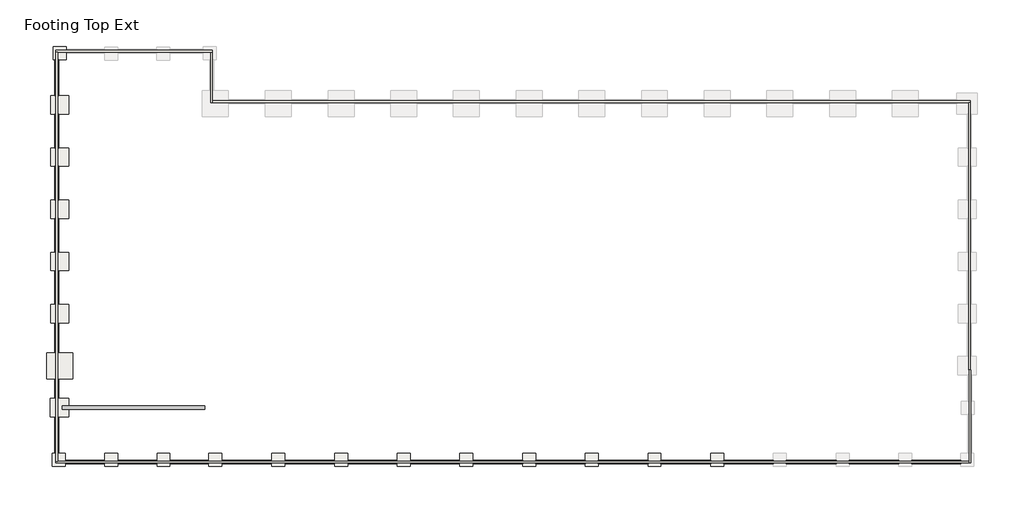
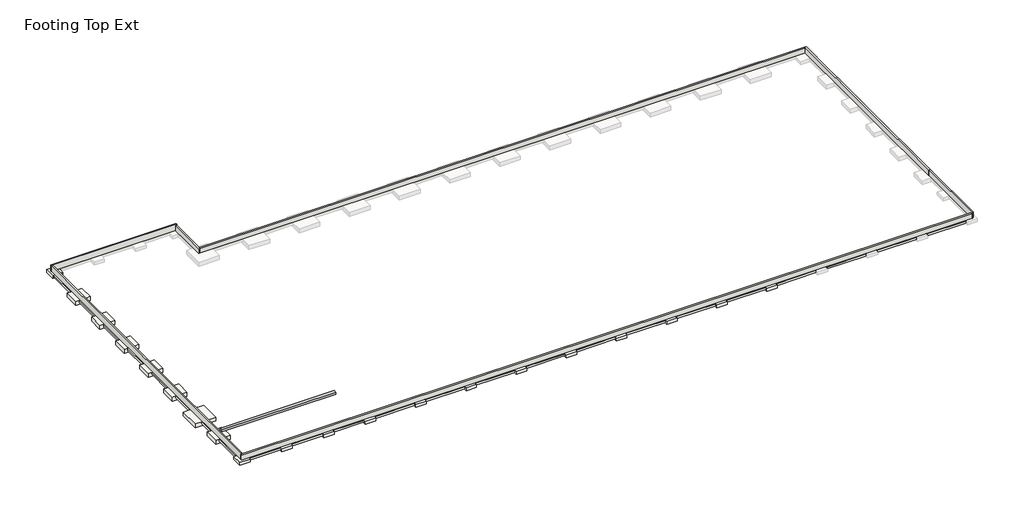
# One storey, part 1 of 2: 20 slabs, 7 walls, 2 footings, 1 beam.
"""IFC4 building model written with IfcOpenShell, lengths in millimetres."""

from ifc_helpers import new_model, si_unit, frame, origin, place, context, project, spatial, polyline, outline, extrude, faceted_brep, element, save

model = new_model("IFC4")

# Units and contexts
model_context = context("Model", 3, world=origin())
ifc_project = project(units=[si_unit("LENGTHUNIT", "METRE", prefix="MILLI")], contexts=[model_context])

# Site, building, storey
site = spatial("IfcSite", under=ifc_project)
building = spatial("IfcBuilding", under=site)
storey = spatial("IfcBuildingStorey", under=building, Name="Footing Top Ext", Elevation=-914.4)

# Beam
placement = place(None, origin())
element("IfcBeam", 1, ObjectType="Concrete-Rectangular Beam : 16 x 12", at=placement, inside=storey, context=model_context, shape_type="SweptSolid", body=[
    extrude(outline(polyline([(321987.9648264, -572404.4391729), (321987.9648264, -572810.8391729), (305258.8898264, -572810.8391729), (305258.8898264, -572404.4391729), (321987.9648264, -572404.4391729)])), frame((0.0, 0.0, -609.6), z_axis=(0.0, 0.0, 1.0), x_axis=(1.0, 0.0, 0.0)), (0.0, 0.0, 1.0), 304.8),
])

# Footings
element("IfcFooting", 2, ObjectType="Bearing Footing - 18\" x 12\"", at=placement, inside=storey, context=model_context, shape_type="SweptSolid", body=[
    extrude(outline(polyline([(305608.1398264, -579216.5913841), (305608.1398264, -578759.3913841), (310230.9398264, -578759.3913841), (310230.9398264, -579216.5913841), (305608.1398264, -579216.5913841)])), frame((0.0, 0.0, -1219.2), z_axis=(0.0, 0.0, 1.0), x_axis=(1.0, 0.0, 0.0)), (0.0, 0.0, 1.0), 304.8),
    extrude(outline(polyline([(311754.9398264, -579216.5913841), (311754.9398264, -578759.3913841), (316361.8648264, -578759.3913841), (316361.8648264, -579216.5913841), (311754.9398264, -579216.5913841)])), frame((0.0, 0.0, -1219.2), z_axis=(0.0, 0.0, 1.0), x_axis=(1.0, 0.0, 0.0)), (0.0, 0.0, 1.0), 304.8),
    extrude(outline(polyline([(317885.8648264, -579216.5913841), (317885.8648264, -578759.3913841), (322457.8648264, -578759.3913841), (322457.8648264, -579216.5913841), (317885.8648264, -579216.5913841)])), frame((0.0, 0.0, -1219.2), z_axis=(0.0, 0.0, 1.0), x_axis=(1.0, 0.0, 0.0)), (0.0, 0.0, 1.0), 304.8),
    extrude(outline(polyline([(323981.8648264, -579216.5913841), (323981.8648264, -578759.3913841), (329839.7398264, -578759.3913841), (329839.7398264, -579216.5913841), (323981.8648264, -579216.5913841)])), frame((0.0, 0.0, -1219.2), z_axis=(0.0, 0.0, 1.0), x_axis=(1.0, 0.0, 0.0)), (0.0, 0.0, 1.0), 304.8),
    extrude(outline(polyline([(331363.7398264, -579216.5913841), (331363.7398264, -578759.3913841), (337193.0398264, -578759.3913841), (337193.0398264, -579216.5913841), (331363.7398264, -579216.5913841)])), frame((0.0, 0.0, -1219.2), z_axis=(0.0, 0.0, 1.0), x_axis=(1.0, 0.0, 0.0)), (0.0, 0.0, 1.0), 304.8),
    extrude(outline(polyline([(338717.0398264, -579216.5913841), (338717.0398264, -578759.3913841), (344546.3398264, -578759.3913841), (344546.3398264, -579216.5913841), (338717.0398264, -579216.5913841)])), frame((0.0, 0.0, -1219.2), z_axis=(0.0, 0.0, 1.0), x_axis=(1.0, 0.0, 0.0)), (0.0, 0.0, 1.0), 304.8),
    extrude(outline(polyline([(346070.3398264, -579216.5913841), (346070.3398264, -578759.3913841), (351899.6398264, -578759.3913841), (351899.6398264, -579216.5913841), (346070.3398264, -579216.5913841)])), frame((0.0, 0.0, -1219.2), z_axis=(0.0, 0.0, 1.0), x_axis=(1.0, 0.0, 0.0)), (0.0, 0.0, 1.0), 304.8),
    extrude(outline(polyline([(353423.6398264, -579216.5913841), (353423.6398264, -578759.3913841), (359252.9398264, -578759.3913841), (359252.9398264, -579216.5913841), (353423.6398264, -579216.5913841)])), frame((0.0, 0.0, -1219.2), z_axis=(0.0, 0.0, 1.0), x_axis=(1.0, 0.0, 0.0)), (0.0, 0.0, 1.0), 304.8),
    extrude(outline(polyline([(360776.9398264, -579216.5913841), (360776.9398264, -578759.3913841), (366606.2398264, -578759.3913841), (366606.2398264, -579216.5913841), (360776.9398264, -579216.5913841)])), frame((0.0, 0.0, -1219.2), z_axis=(0.0, 0.0, 1.0), x_axis=(1.0, 0.0, 0.0)), (0.0, 0.0, 1.0), 304.8),
    extrude(outline(polyline([(368130.2398264, -579216.5913841), (368130.2398264, -578759.3913841), (373959.5398264, -578759.3913841), (373959.5398264, -579216.5913841), (368130.2398264, -579216.5913841)])), frame((0.0, 0.0, -1219.2), z_axis=(0.0, 0.0, 1.0), x_axis=(1.0, 0.0, 0.0)), (0.0, 0.0, 1.0), 304.8),
    extrude(outline(polyline([(375483.5398264, -579216.5913841), (375483.5398264, -578759.3913841), (381312.8398264, -578759.3913841), (381312.8398264, -579216.5913841), (375483.5398264, -579216.5913841)])), frame((0.0, 0.0, -1219.2), z_axis=(0.0, 0.0, 1.0), x_axis=(1.0, 0.0, 0.0)), (0.0, 0.0, 1.0), 304.8),
    extrude(outline(polyline([(382836.8398264, -579216.5913841), (382836.8398264, -578759.3913841), (388666.1398264, -578759.3913841), (388666.1398264, -579216.5913841), (382836.8398264, -579216.5913841)])), frame((0.0, 0.0, -1219.2), z_axis=(0.0, 0.0, 1.0), x_axis=(1.0, 0.0, 0.0)), (0.0, 0.0, 1.0), 304.8),
    extrude(outline(polyline([(390190.1398264, -579216.5913841), (390190.1398264, -578759.3913841), (396019.4398264, -578759.3913841), (396019.4398264, -579216.5913841), (390190.1398264, -579216.5913841)])), frame((0.0, 0.0, -1219.2), z_axis=(0.0, 0.0, 1.0), x_axis=(1.0, 0.0, 0.0)), (0.0, 0.0, 1.0), 304.8),
    extrude(outline(polyline([(397543.4398264, -579216.5913841), (397543.4398264, -578759.3913841), (403372.7398264, -578759.3913841), (403372.7398264, -579216.5913841), (397543.4398264, -579216.5913841)])), frame((0.0, 0.0, -1219.2), z_axis=(0.0, 0.0, 1.0), x_axis=(1.0, 0.0, 0.0)), (0.0, 0.0, 1.0), 304.8),
    extrude(outline(polyline([(404896.7398264, -579216.5913841), (404896.7398264, -578759.3913841), (410675.2398264, -578759.3913841), (410675.2398264, -579216.5913841), (404896.7398264, -579216.5913841)])), frame((0.0, 0.0, -1219.2), z_axis=(0.0, 0.0, 1.0), x_axis=(1.0, 0.0, 0.0)), (0.0, 0.0, 1.0), 304.8),
])
element("IfcFooting", 3, ObjectType="Bearing Footing - 18\" x 12\"", at=placement, inside=storey, context=model_context, shape_type="SweptSolid", body=[
    extrude(outline(polyline([(304369.8898264, -531712.2413841), (304827.0898264, -531712.2413841), (304827.0898264, -535985.7913841), (304369.8898264, -535985.7913841), (304369.8898264, -531712.2413841)])), frame((0.0, 0.0, -1219.2), z_axis=(0.0, 0.0, 1.0), x_axis=(1.0, 0.0, 0.0)), (0.0, 0.0, 1.0), 304.8),
    extrude(outline(polyline([(304369.8898264, -538119.3913841), (304827.0898264, -538119.3913841), (304827.0898264, -542113.5413841), (304369.8898264, -542113.5413841), (304369.8898264, -538119.3913841)])), frame((0.0, 0.0, -1219.2), z_axis=(0.0, 0.0, 1.0), x_axis=(1.0, 0.0, 0.0)), (0.0, 0.0, 1.0), 304.8),
    extrude(outline(polyline([(304369.8898264, -544247.1413841), (304827.0898264, -544247.1413841), (304827.0898264, -548241.2913841), (304369.8898264, -548241.2913841), (304369.8898264, -544247.1413841)])), frame((0.0, 0.0, -1219.2), z_axis=(0.0, 0.0, 1.0), x_axis=(1.0, 0.0, 0.0)), (0.0, 0.0, 1.0), 304.8),
    extrude(outline(polyline([(304369.8898264, -550374.8913841), (304827.0898264, -550374.8913841), (304827.0898264, -554369.0413841), (304369.8898264, -554369.0413841), (304369.8898264, -550374.8913841)])), frame((0.0, 0.0, -1219.2), z_axis=(0.0, 0.0, 1.0), x_axis=(1.0, 0.0, 0.0)), (0.0, 0.0, 1.0), 304.8),
    extrude(outline(polyline([(304369.8898264, -556502.6413841), (304827.0898264, -556502.6413841), (304827.0898264, -560496.7913841), (304369.8898264, -560496.7913841), (304369.8898264, -556502.6413841)])), frame((0.0, 0.0, -1219.2), z_axis=(0.0, 0.0, 1.0), x_axis=(1.0, 0.0, 0.0)), (0.0, 0.0, 1.0), 304.8),
    extrude(outline(polyline([(304369.8898264, -562630.3913841), (304827.0898264, -562630.3913841), (304827.0898264, -566167.3413841), (304369.8898264, -566167.3413841), (304369.8898264, -562630.3913841)])), frame((0.0, 0.0, -1219.2), z_axis=(0.0, 0.0, 1.0), x_axis=(1.0, 0.0, 0.0)), (0.0, 0.0, 1.0), 304.8),
    extrude(outline(polyline([(304369.8898264, -569215.3413841), (304827.0898264, -569215.3413841), (304827.0898264, -571526.7413841), (304369.8898264, -571526.7413841), (304369.8898264, -569215.3413841)])), frame((0.0, 0.0, -1219.2), z_axis=(0.0, 0.0, 1.0), x_axis=(1.0, 0.0, 0.0)), (0.0, 0.0, 1.0), 304.8),
    extrude(outline(polyline([(304369.8898264, -573660.3413841), (304827.0898264, -573660.3413841), (304827.0898264, -577933.8913841), (304369.8898264, -577933.8913841), (304369.8898264, -573660.3413841)])), frame((0.0, 0.0, -1219.2), z_axis=(0.0, 0.0, 1.0), x_axis=(1.0, 0.0, 0.0)), (0.0, 0.0, 1.0), 304.8),
])

# Slabs
element("IfcSlab", 4, ObjectType="Footing-Rectangular : F10", at=placement, inside=storey, context=model_context, shape_type="Brep", body=[
    faceted_brep([(306452.6898264, -566167.3413841, -914.4), (304827.0898264, -566167.3413841, -914.4), (304369.8898264, -566167.3413841, -914.4), (303404.6898264, -566167.3413841, -914.4), (303404.6898264, -569215.3413841, -914.4), (304369.8898264, -569215.3413841, -914.4), (304827.0898264, -569215.3413841, -914.4), (306452.6898264, -569215.3413841, -914.4), (306452.6898264, -566167.3413841, -1524.0), (306452.6898264, -569215.3413841, -1524.0), (303404.6898264, -569215.3413841, -1524.0), (303404.6898264, -566167.3413841, -1524.0)], [[[0, 1, 2, 3, 4, 5, 6, 7]], [[8, 9, 10, 11]], [[3, 2, 1, 0, 8, 11]], [[4, 3, 11, 10]], [[7, 6, 5, 4, 10, 9]], [[0, 7, 9, 8]]]),
])
element("IfcSlab", 5, ObjectType="Footing-Rectangular : F5", at=placement, inside=storey, context=model_context, shape_type="Brep", body=[
    faceted_brep([(305697.0398264, -530188.2413841, -914.4), (304173.0398264, -530188.2413841, -914.4), (304173.0398264, -531712.2413841, -914.4), (304369.8898264, -531712.2413841, -914.4), (304827.0898264, -531712.2413841, -914.4), (305697.0398264, -531712.2413841, -914.4), (305697.0398264, -530975.6413841, -914.4), (305697.0398264, -530518.4413841, -914.4), (305697.0398264, -530188.2413841, -1371.6), (305697.0398264, -531712.2413841, -1371.6), (304173.0398264, -531712.2413841, -1371.6), (304173.0398264, -530188.2413841, -1371.6)], [[[0, 1, 2, 3, 4, 5, 6, 7]], [[8, 9, 10, 11]], [[1, 0, 8, 11]], [[2, 1, 11, 10]], [[5, 4, 3, 2, 10, 9]], [[0, 7, 6, 5, 9, 8]]]),
])
element("IfcSlab", 6, ObjectType="Footing-Rectangular : F5", at=placement, inside=storey, context=model_context, shape_type="Brep", body=[
    faceted_brep([(305608.1398264, -577933.8913841, -914.4), (304827.0898264, -577933.8913841, -914.4), (304369.8898264, -577933.8913841, -914.4), (304084.1398264, -577933.8913841, -914.4), (304084.1398264, -579457.8913841, -914.4), (305608.1398264, -579457.8913841, -914.4), (305608.1398264, -579216.5913841, -914.4), (305608.1398264, -578759.3913841, -914.4), (305608.1398264, -577933.8913841, -1371.6), (305608.1398264, -579457.8913841, -1371.6), (304084.1398264, -579457.8913841, -1371.6), (304084.1398264, -577933.8913841, -1371.6)], [[[0, 1, 2, 3, 4, 5, 6, 7]], [[8, 9, 10, 11]], [[3, 2, 1, 0, 8, 11]], [[4, 3, 11, 10]], [[5, 4, 10, 9]], [[0, 7, 6, 5, 9, 8]]]),
])
element("IfcSlab", 7, ObjectType="Footing-Rectangular : F5", at=placement, inside=storey, context=model_context, shape_type="Brep", body=[
    faceted_brep([(311754.9398264, -577927.5413841, -914.4), (310230.9398264, -577927.5413841, -914.4), (310230.9398264, -578759.3913841, -914.4), (310230.9398264, -579216.5913841, -914.4), (310230.9398264, -579451.5413841, -914.4), (311754.9398264, -579451.5413841, -914.4), (311754.9398264, -579216.5913841, -914.4), (311754.9398264, -578759.3913841, -914.4), (311754.9398264, -577927.5413841, -1371.6), (311754.9398264, -579451.5413841, -1371.6), (310230.9398264, -579451.5413841, -1371.6), (310230.9398264, -577927.5413841, -1371.6)], [[[0, 1, 2, 3, 4, 5, 6, 7]], [[8, 9, 10, 11]], [[1, 0, 8, 11]], [[4, 3, 2, 1, 11, 10]], [[5, 4, 10, 9]], [[0, 7, 6, 5, 9, 8]]]),
])
element("IfcSlab", 8, ObjectType="Footing-Rectangular : F5", at=placement, inside=storey, context=model_context, shape_type="Brep", body=[
    faceted_brep([(317885.8648264, -577971.9913841, -914.4), (316361.8648264, -577971.9913841, -914.4), (316361.8648264, -578759.3913841, -914.4), (316361.8648264, -579216.5913841, -914.4), (316361.8648264, -579495.9913841, -914.4), (317885.8648264, -579495.9913841, -914.4), (317885.8648264, -579216.5913841, -914.4), (317885.8648264, -578759.3913841, -914.4), (317885.8648264, -577971.9913841, -1371.6), (317885.8648264, -579495.9913841, -1371.6), (316361.8648264, -579495.9913841, -1371.6), (316361.8648264, -577971.9913841, -1371.6)], [[[0, 1, 2, 3, 4, 5, 6, 7]], [[8, 9, 10, 11]], [[1, 0, 8, 11]], [[4, 3, 2, 1, 11, 10]], [[5, 4, 10, 9]], [[0, 7, 6, 5, 9, 8]]]),
])
element("IfcSlab", 9, ObjectType="Footing-Rectangular : F5", at=placement, inside=storey, context=model_context, shape_type="Brep", body=[
    faceted_brep([(323981.8648264, -577971.9913841, -914.4), (322457.8648264, -577971.9913841, -914.4), (322457.8648264, -578759.3913841, -914.4), (322457.8648264, -579216.5913841, -914.4), (322457.8648264, -579495.9913841, -914.4), (323981.8648264, -579495.9913841, -914.4), (323981.8648264, -579216.5913841, -914.4), (323981.8648264, -578759.3913841, -914.4), (323981.8648264, -577971.9913841, -1371.6), (323981.8648264, -579495.9913841, -1371.6), (322457.8648264, -579495.9913841, -1371.6), (322457.8648264, -577971.9913841, -1371.6)], [[[0, 1, 2, 3, 4, 5, 6, 7]], [[8, 9, 10, 11]], [[1, 0, 8, 11]], [[4, 3, 2, 1, 11, 10]], [[5, 4, 10, 9]], [[0, 7, 6, 5, 9, 8]]]),
])
element("IfcSlab", 10, ObjectType="Footing-Rectangular : F5", at=placement, inside=storey, context=model_context, shape_type="Brep", body=[
    faceted_brep([(331363.7398264, -577978.3413841, -914.4), (329839.7398264, -577978.3413841, -914.4), (329839.7398264, -578759.3913841, -914.4), (329839.7398264, -579216.5913841, -914.4), (329839.7398264, -579502.3413841, -914.4), (331363.7398264, -579502.3413841, -914.4), (331363.7398264, -579216.5913841, -914.4), (331363.7398264, -578759.3913841, -914.4), (331363.7398264, -577978.3413841, -1371.6), (331363.7398264, -579502.3413841, -1371.6), (329839.7398264, -579502.3413841, -1371.6), (329839.7398264, -577978.3413841, -1371.6)], [[[0, 1, 2, 3, 4, 5, 6, 7]], [[8, 9, 10, 11]], [[1, 0, 8, 11]], [[4, 3, 2, 1, 11, 10]], [[5, 4, 10, 9]], [[0, 7, 6, 5, 9, 8]]]),
])
element("IfcSlab", 11, ObjectType="Footing-Rectangular : F5", at=placement, inside=storey, context=model_context, shape_type="Brep", body=[
    faceted_brep([(338717.0398264, -577978.3413841, -914.4), (337193.0398264, -577978.3413841, -914.4), (337193.0398264, -578759.3913841, -914.4), (337193.0398264, -579216.5913841, -914.4), (337193.0398264, -579502.3413841, -914.4), (338717.0398264, -579502.3413841, -914.4), (338717.0398264, -579216.5913841, -914.4), (338717.0398264, -578759.3913841, -914.4), (338717.0398264, -577978.3413841, -1371.6), (338717.0398264, -579502.3413841, -1371.6), (337193.0398264, -579502.3413841, -1371.6), (337193.0398264, -577978.3413841, -1371.6)], [[[0, 1, 2, 3, 4, 5, 6, 7]], [[8, 9, 10, 11]], [[1, 0, 8, 11]], [[4, 3, 2, 1, 11, 10]], [[5, 4, 10, 9]], [[0, 7, 6, 5, 9, 8]]]),
])
element("IfcSlab", 12, ObjectType="Footing-Rectangular : F5", at=placement, inside=storey, context=model_context, shape_type="Brep", body=[
    faceted_brep([(346070.3398264, -577978.3413841, -914.4), (344546.3398264, -577978.3413841, -914.4), (344546.3398264, -578759.3913841, -914.4), (344546.3398264, -579216.5913841, -914.4), (344546.3398264, -579502.3413841, -914.4), (346070.3398264, -579502.3413841, -914.4), (346070.3398264, -579216.5913841, -914.4), (346070.3398264, -578759.3913841, -914.4), (346070.3398264, -577978.3413841, -1371.6), (346070.3398264, -579502.3413841, -1371.6), (344546.3398264, -579502.3413841, -1371.6), (344546.3398264, -577978.3413841, -1371.6)], [[[0, 1, 2, 3, 4, 5, 6, 7]], [[8, 9, 10, 11]], [[1, 0, 8, 11]], [[4, 3, 2, 1, 11, 10]], [[5, 4, 10, 9]], [[0, 7, 6, 5, 9, 8]]]),
])
element("IfcSlab", 13, ObjectType="Footing-Rectangular : F5", at=placement, inside=storey, context=model_context, shape_type="Brep", body=[
    faceted_brep([(353423.6398264, -577978.3413841, -914.4), (351899.6398264, -577978.3413841, -914.4), (351899.6398264, -578759.3913841, -914.4), (351899.6398264, -579216.5913841, -914.4), (351899.6398264, -579502.3413841, -914.4), (353423.6398264, -579502.3413841, -914.4), (353423.6398264, -579216.5913841, -914.4), (353423.6398264, -578759.3913841, -914.4), (353423.6398264, -577978.3413841, -1371.6), (353423.6398264, -579502.3413841, -1371.6), (351899.6398264, -579502.3413841, -1371.6), (351899.6398264, -577978.3413841, -1371.6)], [[[0, 1, 2, 3, 4, 5, 6, 7]], [[8, 9, 10, 11]], [[1, 0, 8, 11]], [[4, 3, 2, 1, 11, 10]], [[5, 4, 10, 9]], [[0, 7, 6, 5, 9, 8]]]),
])
element("IfcSlab", 14, ObjectType="Footing-Rectangular : F5", at=placement, inside=storey, context=model_context, shape_type="Brep", body=[
    faceted_brep([(360776.9398264, -577978.3413841, -914.4), (359252.9398264, -577978.3413841, -914.4), (359252.9398264, -578759.3913841, -914.4), (359252.9398264, -579216.5913841, -914.4), (359252.9398264, -579502.3413841, -914.4), (360776.9398264, -579502.3413841, -914.4), (360776.9398264, -579216.5913841, -914.4), (360776.9398264, -578759.3913841, -914.4), (360776.9398264, -577978.3413841, -1371.6), (360776.9398264, -579502.3413841, -1371.6), (359252.9398264, -579502.3413841, -1371.6), (359252.9398264, -577978.3413841, -1371.6)], [[[0, 1, 2, 3, 4, 5, 6, 7]], [[8, 9, 10, 11]], [[1, 0, 8, 11]], [[4, 3, 2, 1, 11, 10]], [[5, 4, 10, 9]], [[0, 7, 6, 5, 9, 8]]]),
])
element("IfcSlab", 15, ObjectType="Footing-Rectangular : F5", at=placement, inside=storey, context=model_context, shape_type="Brep", body=[
    faceted_brep([(368130.2398264, -577978.3413841, -914.4), (366606.2398264, -577978.3413841, -914.4), (366606.2398264, -578759.3913841, -914.4), (366606.2398264, -579216.5913841, -914.4), (366606.2398264, -579502.3413841, -914.4), (368130.2398264, -579502.3413841, -914.4), (368130.2398264, -579216.5913841, -914.4), (368130.2398264, -578759.3913841, -914.4), (368130.2398264, -577978.3413841, -1371.6), (368130.2398264, -579502.3413841, -1371.6), (366606.2398264, -579502.3413841, -1371.6), (366606.2398264, -577978.3413841, -1371.6)], [[[0, 1, 2, 3, 4, 5, 6, 7]], [[8, 9, 10, 11]], [[1, 0, 8, 11]], [[4, 3, 2, 1, 11, 10]], [[5, 4, 10, 9]], [[0, 7, 6, 5, 9, 8]]]),
])
element("IfcSlab", 16, ObjectType="Footing-Rectangular : F5", at=placement, inside=storey, context=model_context, shape_type="Brep", body=[
    faceted_brep([(375483.5398264, -577978.3413841, -914.4), (373959.5398264, -577978.3413841, -914.4), (373959.5398264, -578759.3913841, -914.4), (373959.5398264, -579216.5913841, -914.4), (373959.5398264, -579502.3413841, -914.4), (375483.5398264, -579502.3413841, -914.4), (375483.5398264, -579216.5913841, -914.4), (375483.5398264, -578759.3913841, -914.4), (375483.5398264, -577978.3413841, -1371.6), (375483.5398264, -579502.3413841, -1371.6), (373959.5398264, -579502.3413841, -1371.6), (373959.5398264, -577978.3413841, -1371.6)], [[[0, 1, 2, 3, 4, 5, 6, 7]], [[8, 9, 10, 11]], [[1, 0, 8, 11]], [[4, 3, 2, 1, 11, 10]], [[5, 4, 10, 9]], [[0, 7, 6, 5, 9, 8]]]),
])
element("IfcSlab", 17, ObjectType="Footing-Rectangular : F5", at=placement, inside=storey, context=model_context, shape_type="Brep", body=[
    faceted_brep([(382836.8398264, -577978.3413841, -914.4), (381312.8398264, -577978.3413841, -914.4), (381312.8398264, -578759.3913841, -914.4), (381312.8398264, -579216.5913841, -914.4), (381312.8398264, -579502.3413841, -914.4), (382836.8398264, -579502.3413841, -914.4), (382836.8398264, -579216.5913841, -914.4), (382836.8398264, -578759.3913841, -914.4), (382836.8398264, -577978.3413841, -1371.6), (382836.8398264, -579502.3413841, -1371.6), (381312.8398264, -579502.3413841, -1371.6), (381312.8398264, -577978.3413841, -1371.6)], [[[0, 1, 2, 3, 4, 5, 6, 7]], [[8, 9, 10, 11]], [[1, 0, 8, 11]], [[4, 3, 2, 1, 11, 10]], [[5, 4, 10, 9]], [[0, 7, 6, 5, 9, 8]]]),
])
element("IfcSlab", 18, ObjectType="Footing-Rectangular : F7", at=placement, inside=storey, context=model_context, shape_type="Brep", body=[
    faceted_brep([(306020.8898264, -535985.7913841, -914.4), (304827.0898264, -535985.7913841, -914.4), (304369.8898264, -535985.7913841, -914.4), (303887.2898264, -535985.7913841, -914.4), (303887.2898264, -538119.3913841, -914.4), (304369.8898264, -538119.3913841, -914.4), (304827.0898264, -538119.3913841, -914.4), (306020.8898264, -538119.3913841, -914.4), (306020.8898264, -535985.7913841, -1524.0), (306020.8898264, -538119.3913841, -1524.0), (303887.2898264, -538119.3913841, -1524.0), (303887.2898264, -535985.7913841, -1524.0)], [[[0, 1, 2, 3, 4, 5, 6, 7]], [[8, 9, 10, 11]], [[3, 2, 1, 0, 8, 11]], [[4, 3, 11, 10]], [[7, 6, 5, 4, 10, 9]], [[0, 7, 9, 8]]]),
])
element("IfcSlab", 19, ObjectType="Footing-Rectangular : F7", at=placement, inside=storey, context=model_context, shape_type="Brep", body=[
    faceted_brep([(306020.8898264, -542113.5413841, -914.4), (304827.0898264, -542113.5413841, -914.4), (304369.8898264, -542113.5413841, -914.4), (303887.2898264, -542113.5413841, -914.4), (303887.2898264, -544247.1413841, -914.4), (304369.8898264, -544247.1413841, -914.4), (304827.0898264, -544247.1413841, -914.4), (306020.8898264, -544247.1413841, -914.4), (306020.8898264, -542113.5413841, -1524.0), (306020.8898264, -544247.1413841, -1524.0), (303887.2898264, -544247.1413841, -1524.0), (303887.2898264, -542113.5413841, -1524.0)], [[[0, 1, 2, 3, 4, 5, 6, 7]], [[8, 9, 10, 11]], [[3, 2, 1, 0, 8, 11]], [[4, 3, 11, 10]], [[7, 6, 5, 4, 10, 9]], [[0, 7, 9, 8]]]),
])
element("IfcSlab", 20, ObjectType="Footing-Rectangular : F7", at=placement, inside=storey, context=model_context, shape_type="Brep", body=[
    faceted_brep([(306020.8898264, -548241.2913841, -914.4), (304827.0898264, -548241.2913841, -914.4), (304369.8898264, -548241.2913841, -914.4), (303887.2898264, -548241.2913841, -914.4), (303887.2898264, -550374.8913841, -914.4), (304369.8898264, -550374.8913841, -914.4), (304827.0898264, -550374.8913841, -914.4), (306020.8898264, -550374.8913841, -914.4), (306020.8898264, -548241.2913841, -1524.0), (306020.8898264, -550374.8913841, -1524.0), (303887.2898264, -550374.8913841, -1524.0), (303887.2898264, -548241.2913841, -1524.0)], [[[0, 1, 2, 3, 4, 5, 6, 7]], [[8, 9, 10, 11]], [[3, 2, 1, 0, 8, 11]], [[4, 3, 11, 10]], [[7, 6, 5, 4, 10, 9]], [[0, 7, 9, 8]]]),
])
element("IfcSlab", 21, ObjectType="Footing-Rectangular : F7", at=placement, inside=storey, context=model_context, shape_type="Brep", body=[
    faceted_brep([(306020.8898264, -554369.0413841, -914.4), (304827.0898264, -554369.0413841, -914.4), (304369.8898264, -554369.0413841, -914.4), (303887.2898264, -554369.0413841, -914.4), (303887.2898264, -556502.6413841, -914.4), (304369.8898264, -556502.6413841, -914.4), (304827.0898264, -556502.6413841, -914.4), (306020.8898264, -556502.6413841, -914.4), (306020.8898264, -554369.0413841, -1524.0), (306020.8898264, -556502.6413841, -1524.0), (303887.2898264, -556502.6413841, -1524.0), (303887.2898264, -554369.0413841, -1524.0)], [[[0, 1, 2, 3, 4, 5, 6, 7]], [[8, 9, 10, 11]], [[3, 2, 1, 0, 8, 11]], [[4, 3, 11, 10]], [[7, 6, 5, 4, 10, 9]], [[0, 7, 9, 8]]]),
])
element("IfcSlab", 22, ObjectType="Footing-Rectangular : F7", at=placement, inside=storey, context=model_context, shape_type="Brep", body=[
    faceted_brep([(306020.8898264, -560496.7913841, -914.4), (304827.0898264, -560496.7913841, -914.4), (304369.8898264, -560496.7913841, -914.4), (303887.2898264, -560496.7913841, -914.4), (303887.2898264, -562630.3913841, -914.4), (304369.8898264, -562630.3913841, -914.4), (304827.0898264, -562630.3913841, -914.4), (306020.8898264, -562630.3913841, -914.4), (306020.8898264, -560496.7913841, -1524.0), (306020.8898264, -562630.3913841, -1524.0), (303887.2898264, -562630.3913841, -1524.0), (303887.2898264, -560496.7913841, -1524.0)], [[[0, 1, 2, 3, 4, 5, 6, 7]], [[8, 9, 10, 11]], [[3, 2, 1, 0, 8, 11]], [[4, 3, 11, 10]], [[7, 6, 5, 4, 10, 9]], [[0, 7, 9, 8]]]),
])
element("IfcSlab", 23, ObjectType="Footing-Rectangular : F7", at=placement, inside=storey, context=model_context, shape_type="Brep", body=[
    faceted_brep([(305995.4898264, -571526.7413841, -914.4), (304827.0898264, -571526.7413841, -914.4), (304369.8898264, -571526.7413841, -914.4), (303861.8898264, -571526.7413841, -914.4), (303861.8898264, -573660.3413841, -914.4), (304369.8898264, -573660.3413841, -914.4), (304827.0898264, -573660.3413841, -914.4), (305995.4898264, -573660.3413841, -914.4), (305995.4898264, -571526.7413841, -1524.0), (305995.4898264, -573660.3413841, -1524.0), (303861.8898264, -573660.3413841, -1524.0), (303861.8898264, -571526.7413841, -1524.0)], [[[0, 1, 2, 3, 4, 5, 6, 7]], [[8, 9, 10, 11]], [[3, 2, 1, 0, 8, 11]], [[4, 3, 11, 10]], [[7, 6, 5, 4, 10, 9]], [[0, 7, 9, 8]]]),
])

# Walls
element("IfcWall", 24, ObjectType="Frost Wall - 8\" Concrete", at=placement, inside=storey, context=model_context, shape_type="Brep", body=[
    faceted_brep([(304496.8898264, -530848.6413841, -914.4), (304681.0398264, -530848.6413841, -914.4), (322664.2398264, -530848.6413841, -914.4), (322867.4398264, -530848.6413841, -914.4), (322867.4398264, -530848.6413841, -152.4), (322867.4398264, -530848.6413841, 0.0), (304496.8898264, -530848.6413841, 0.0), (304496.8898264, -530848.6413841, -152.4), (304496.8898264, -530645.4413841, -914.4), (304496.8898264, -530645.4413841, 0.0), (322867.4398264, -530645.4413841, 0.0), (322867.4398264, -530645.4413841, -914.4)], [[[0, 1, 2, 3, 4, 5, 6, 7]], [[8, 9, 10, 11]], [[3, 2, 1, 0, 8, 11]], [[6, 5, 10, 9]], [[5, 4, 3, 11, 10]], [[0, 7, 6, 9, 8]]]),
])
element("IfcWall", 25, ObjectType="Frost Wall - 8\" Concrete", at=placement, inside=storey, context=model_context, shape_type="Brep", body=[
    faceted_brep([(322664.2398264, -530848.6413841, -914.4), (322664.2398264, -536760.4913841, -914.4), (322664.2398264, -536760.4913841, -152.4), (322664.2398264, -536088.5033331, -152.4), (322664.2398264, -530848.6413841, -152.4), (322867.4398264, -536760.4913841, -914.4), (322867.4398264, -536557.2913841, -914.4), (322867.4398264, -530848.6413841, -914.4), (322867.4398264, -530848.6413841, -152.4), (322867.4398264, -536557.2913841, -152.4), (322867.4398264, -536760.4913841, -152.4)], [[[0, 1, 2, 3, 4]], [[5, 6, 7, 8, 9, 10]], [[1, 0, 7, 6, 5]], [[7, 0, 4, 8]], [[1, 5, 10, 2]], [[3, 2, 10, 9, 8, 4]]]),
])
element("IfcWall", 26, ObjectType="Frost Wall - 8\" Concrete", at=placement, inside=storey, context=model_context, shape_type="Brep", body=[
    faceted_brep([(322867.4398264, -536760.4913841, -914.4), (411564.2398264, -536760.4913841, -914.4), (411767.4398264, -536760.4913841, -914.4), (411767.4398264, -536760.4913841, -152.4), (322867.4398264, -536760.4913841, -152.4), (411767.4398264, -536557.2913841, -914.4), (322867.4398264, -536557.2913841, -914.4), (322867.4398264, -536557.2913841, -152.4), (411767.4398264, -536557.2913841, -152.4)], [[[0, 1, 2, 3, 4]], [[5, 6, 7, 8]], [[2, 1, 0, 6, 5]], [[6, 0, 4, 7]], [[2, 5, 8, 3]], [[4, 3, 8, 7]]]),
])
element("IfcWall", 27, ObjectType="Frost Wall - 8\" Concrete", at=placement, inside=storey, context=model_context, shape_type="Brep", body=[
    faceted_brep([(411564.2398264, -536760.4913841, -914.4), (411564.2398264, -568186.6413841, -914.4), (411564.2398264, -568186.6413841, 0.0), (411564.2398264, -536760.4913841, 0.0), (411767.4398264, -536760.4913841, -914.4), (411767.4398264, -536760.4913841, -152.4), (411767.4398264, -536760.4913841, 0.0), (411767.4398264, -568186.6413841, 0.0), (411767.4398264, -568186.6413841, -914.4), (411615.0398264, -568186.6413841, -914.4), (411615.0398264, -568186.6413841, 0.0)], [[[0, 1, 2, 3]], [[4, 5, 6, 7, 8]], [[1, 0, 4, 8, 9]], [[2, 1, 9, 8, 7, 10]], [[3, 2, 10, 7, 6]], [[0, 3, 6, 5, 4]]]),
])
element("IfcWall", 28, ObjectType="Frost Wall - 8\" Concrete", at=placement, inside=storey, context=model_context, shape_type="Brep", body=[
    faceted_brep([(411615.0398264, -578886.3913841, -914.4), (304700.0898264, -578886.3913841, -914.4), (304496.8898264, -578886.3913841, -914.4), (304496.8898264, -578886.3913841, -152.4), (304700.0898264, -578886.3913841, -152.4), (411615.0398264, -578886.3913841, -152.4), (304496.8898264, -579089.5913841, -914.4), (411615.0398264, -579089.5913841, -914.4), (411615.0398264, -579089.5913841, -152.4), (304496.8898264, -579089.5913841, -152.4)], [[[0, 1, 2, 3, 4, 5]], [[6, 7, 8, 9]], [[2, 1, 0, 7, 6]], [[7, 0, 5, 8]], [[2, 6, 9, 3]], [[5, 4, 3, 9, 8]]]),
])
element("IfcWall", 29, ObjectType="Frost Wall - 8\" Concrete", at=placement, inside=storey, context=model_context, shape_type="Brep", body=[
    faceted_brep([(304700.0898264, -578886.3913841, -914.4), (304700.0898264, -530848.6413841, -914.4), (304700.0898264, -530848.6413841, 0.0), (304700.0898264, -578886.3913841, 0.0), (304496.8898264, -578886.3913841, -914.4), (304496.8898264, -578886.3913841, -152.4), (304496.8898264, -578886.3913841, 0.0), (304496.8898264, -530848.6413841, 0.0), (304496.8898264, -530848.6413841, -914.4)], [[[0, 1, 2, 3]], [[4, 5, 6, 7, 8]], [[1, 0, 4, 8]], [[3, 2, 7, 6]], [[2, 1, 8, 7]], [[0, 3, 6, 5, 4]]]),
])
element("IfcWall", 30, ObjectType="Frost Wall - 8\" Concrete", at=placement, inside=storey, context=model_context, shape_type="Brep", body=[
    faceted_brep([(411615.0398264, -568186.6413841, -914.4), (411615.0398264, -578886.3913841, -914.4), (411615.0398264, -579089.5913841, -914.4), (411615.0398264, -579089.5913841, -152.4), (411615.0398264, -579089.5913841, 0.0), (411615.0398264, -568186.6413841, 0.0), (411818.2398264, -568186.6413841, -914.4), (411818.2398264, -568186.6413841, 0.0), (411818.2398264, -579089.5913841, 0.0), (411818.2398264, -579089.5913841, -914.4), (411767.4398264, -568186.6413841, -914.4), (411767.4398264, -568186.6413841, 0.0)], [[[0, 1, 2, 3, 4, 5]], [[6, 7, 8, 9]], [[2, 1, 0, 10, 6, 9]], [[5, 4, 8, 7, 11]], [[0, 5, 11, 7, 6, 10]], [[4, 3, 2, 9, 8]]]),
])

save(model, "model.ifc")

# Revit data of these elements
# Project information
#   Project Issue Date = "Issue Date"
#   Project Status = "Project Status"
#   Client Name = "Xcel"
#   Project Address = "Enter address here"
#   Project Name = "Sports Complex"
#   Project Number = "Project Number"
# Grids (mm)
#   "1-7": line (367368.24, -472874.843) -> (367368.24, -606417.413)
#   "1-6": line (374721.54, -472874.843) -> (374721.54, -606417.413)
#   "2-12": line (330601.74, -475922.843) -> (330601.74, -609465.413)
#   "2": line (330601.74, -462514.089) -> (330601.74, -614425.444)
#   "3": line (337955.04, -462514.089) -> (337955.04, -614425.444)
#   "4": line (310992.94, -462514.089) -> (310992.94, -614425.444)
#   "5": line (317120.69, -462514.089) -> (317120.69, -614425.444)
#   "6": line (304788.99, -466694.458) -> (304788.99, -614353.824)
#   "7": line (304585.79, -462514.089) -> (304585.79, -614425.444)
#   "8": line (323527.84, -456865.657) -> (323527.84, -614425.444)
#   "9": line (323324.64, -458611.498) -> (323324.64, -614425.444)
#   "10": line (323121.44, -459359.716) -> (323121.44, -614425.444)
#   "1-13.G ALT": line (322867.44, -459359.716) -> (322867.44, -614425.444)
#   "12": line (330601.74, -466694.458) -> (330601.74, -617473.444)
#   "13": line (337955.04, -466694.458) -> (337955.04, -617473.444)
#   "14": line (323324.64, -466694.458) -> (323324.64, -616559.044)
#   "3-D ALT": line (322664.24, -456865.657) -> (322664.24, -614425.444)
#   "3-D.G ALT": line (322867.44, -458611.498) -> (322867.44, -614425.444)
#   "1-12": line (330601.74, -472874.843) -> (330601.74, -606417.413)
#   "1-11": line (337955.04, -472874.843) -> (337955.04, -606417.413)
#   "1-10": line (345308.34, -472874.843) -> (345308.34, -606417.413)
#   "1-9": line (352661.64, -472874.843) -> (352661.64, -606417.413)
#   "1-8": line (360014.94, -472874.843) -> (360014.94, -606417.413)
#   "3-8": line (243887.399, -537052.591) -> (490605.763, -537052.591)
#   "3-3": line (243887.399, -567691.341) -> (490605.763, -567691.341)
#   "3-7": line (243887.399, -543180.341) -> (426856.7, -543180.341)
#   "3-6": line (243887.399, -549308.091) -> (426856.7, -549308.091)
#   "1-5": line (382074.84, -472874.843) -> (382074.84, -606417.413)
#   "1-4": line (389428.14, -472874.843) -> (389428.14, -606417.413)
#   "1-3": line (396781.44, -472874.843) -> (396781.44, -606417.413)
#   "1-2": line (404134.74, -472874.843) -> (404134.74, -606417.413)
#   "3-5": line (243887.399, -555435.841) -> (426856.7, -555435.841)
#   "3-4": line (243887.399, -561563.591) -> (426856.7, -561563.591)
#   "3-2": line (243887.399, -572593.541) -> (490605.763, -572593.541)
#   "3-B": line (310992.94, -472874.843) -> (310992.94, -606417.413)
#   "3-C": line (317120.69, -472874.843) -> (317120.69, -606417.413)
#   "3-1": line (243887.399, -578797.491) -> (490605.763, -578797.491)
#   "3-1.G": line (243887.399, -579000.691) -> (490605.763, -579000.691)
#   "3-E": line (323324.64, -472874.843) -> (323324.64, -606417.413)
#   "3-A": line (304788.99, -472803.223) -> (304788.99, -606345.792)
#   "3-A.G": line (304585.79, -472874.843) -> (304585.79, -606417.413)
#   "3-9": line (243887.399, -530848.641) -> (490605.763, -530848.641)
#   "3-9.G": line (243887.399, -530645.441) -> (490605.763, -530645.441)
#   "3-E.G": line (323527.84, -472874.843) -> (323527.84, -606417.413)
#   "3-3.G": line (243887.399, -567488.141) -> (490605.763, -567488.141)
#   "1-1G": line (411767.44, -472874.843) -> (411767.44, -606417.413)
#   "2-1": line (411564.24, -472874.843) -> (411564.24, -606417.413)
#   "1-1.G": line (411513.44, -472874.843) -> (411513.44, -606417.413)
#   "1-13": line (323121.44, -472874.843) -> (323121.44, -606417.413)
#   "1-A": line (243887.399, -567932.641) -> (426856.7, -567932.641)
#   "1-A.G": line (243887.399, -568186.641) -> (426856.7, -568186.641)
#   "1-13.G": line (322867.44, -472874.843) -> (322867.44, -606417.413)
#   "3-D": line (322664.24, -472874.843) -> (322664.24, -606417.413)
#   "1-F": line (243887.399, -536811.291) -> (426856.7, -536811.291)
#   "1-F.G": line (243887.399, -536557.291) -> (426856.7, -536557.291)
#   "3-D.G": line (322867.44, -472874.843) -> (322867.44, -606417.413)
#   "1-E": line (240890.199, -543180.341) -> (423859.5, -543180.341)
#   "1-D": line (240890.199, -549308.091) -> (423859.5, -549308.091)
#   "1-C": line (240890.199, -555435.841) -> (423859.5, -555435.841)
#   "1-B": line (240890.199, -561563.591) -> (423859.5, -561563.591)
#   "2-B": line (239924.999, -572593.541) -> (486643.363, -572593.541)
#   "2-A": line (240534.599, -578797.491) -> (487252.963, -578797.491)
#   "2-A.G": line (240534.599, -579000.691) -> (487252.963, -579000.691)
#   "2-7": line (367368.24, -475922.843) -> (367368.24, -609465.413)
#   "2-6": line (374721.54, -475922.843) -> (374721.54, -609465.413)
#   "2-5": line (382074.84, -475922.843) -> (382074.84, -609465.413)
#   "2-4": line (389428.14, -475922.843) -> (389428.14, -609465.413)
#   "2-3": line (396781.44, -475922.843) -> (396781.44, -609465.413)
#   "2-11": line (337955.04, -475922.843) -> (337955.04, -609465.413)
#   "2-10": line (345308.34, -475922.843) -> (345308.34, -609465.413)
#   "2-9": line (352661.64, -475922.843) -> (352661.64, -609465.413)
#   "2-8": line (360014.94, -475922.843) -> (360014.94, -609465.413)
#   "2-2": line (404134.74, -475922.843) -> (404134.74, -609465.413)
#   "2-13": line (323324.64, -475008.443) -> (323324.64, -608551.013)
#   "2-1G": line (411767.44, -476684.843) -> (411767.44, -610227.413)
#   "2-C": line (241753.799, -567932.641) -> (424723.1, -567932.641)
#   "2-3.G": line (396578.24, -475922.843) -> (396578.24, -609465.413)
# Type "Concrete-Rectangular Beam : 16 x 12"
#   Assembly Code = "B10"
#   Length [instance default] = 5' - 0"
#   b = 1' - 4"
#   h = 1' - 0"
#   Structural Material [instance default] = Concrete, Cast-in-Place gray
# Type "Bearing Footing - 18\" x 12\""
#   Assembly Code = "A1010110"
# Type "Footing-Rectangular : F10"
#   Assembly Code = "A1010100"
#   Width = 10' - 0"
#   Length = 10' - 0"
#   Thickness = 2' - 0"
#   Structural Material [instance default] = Concrete, Cast-in-Place gray
# Type "Footing-Rectangular : F5"
#   Assembly Code = "A1010100"
#   Width = 5' - 0"
#   Length = 5' - 0"
#   Thickness = 1' - 6"
#   Structural Material [instance default] = Concrete, Cast-in-Place gray
# Type "Footing-Rectangular : F7"
#   Assembly Code = "A1010100"
#   Width = 7' - 0"
#   Length = 7' - 0"
#   Thickness = 2' - 0"
#   Structural Material [instance default] = Concrete, Cast-in-Place gray
# Type "Frost Wall - 8\" Concrete"
#   Assembly Code = "B2010"
#   Width = 0' - 8"
#   Layers, outside or top first: 0' - 8" "Concrete, Cast-in-Place gray" (function 1)
# Element 1 (IfcBeam, "Concrete-Rectangular Beam : 16 x 12")
#   Comments = ""
#   Structural Material = Concrete, Cast-in-Place gray
#   Phase Created = New Construction
#   Materials on its faces: "Concrete, Cast-in-Place gray"
# Elements 2, 3 (IfcFooting, "Bearing Footing - 18\" x 12\"")
#   Phase Created = New Construction
#   Materials on its faces: "Concrete, Cast-in-Place gray"
# Element 4 (IfcSlab, "Footing-Rectangular : F10")
#   Comments = ""
#   Structural Material = Concrete, Cast-in-Place gray
#   Phase Created = New Construction
#   Materials on its faces: "Concrete, Cast-in-Place gray"
# Elements 5, 6, 7, 8, 9, 10, 11, 12, 13, 14, 15, 16, 17 (IfcSlab, "Footing-Rectangular : F5")
#   Comments = ""
#   Structural Material = Concrete, Cast-in-Place gray
#   Phase Created = New Construction
#   Materials on its faces: "Concrete, Cast-in-Place gray"
# Elements 18, 19, 20, 21, 22, 23 (IfcSlab, "Footing-Rectangular : F7")
#   Comments = ""
#   Structural Material = Concrete, Cast-in-Place gray
#   Phase Created = New Construction
#   Materials on its faces: "Concrete, Cast-in-Place gray"
# Elements 24, 25, 26, 27, 28, 29, 30 (IfcWall, "Frost Wall - 8\" Concrete")
#   Comments = ""
#   Top Offset = 0' - 0"
#   Base Offset = 0' - 0"
#   wall height = 3' - 0"
#   Phase Created = New Construction
#   Base Constraint = Footing Top Ext
#   Top Constraint = Level 1
#   Materials on its faces: "Concrete, Cast-in-Place gray"
# Materials
#   "Concrete, Cast-in-Place gray": class "Concrete", colour RGB 192 192 192, transparency 0, Description = "Cast-in-place concrete", Cost = 0
